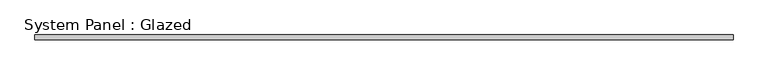
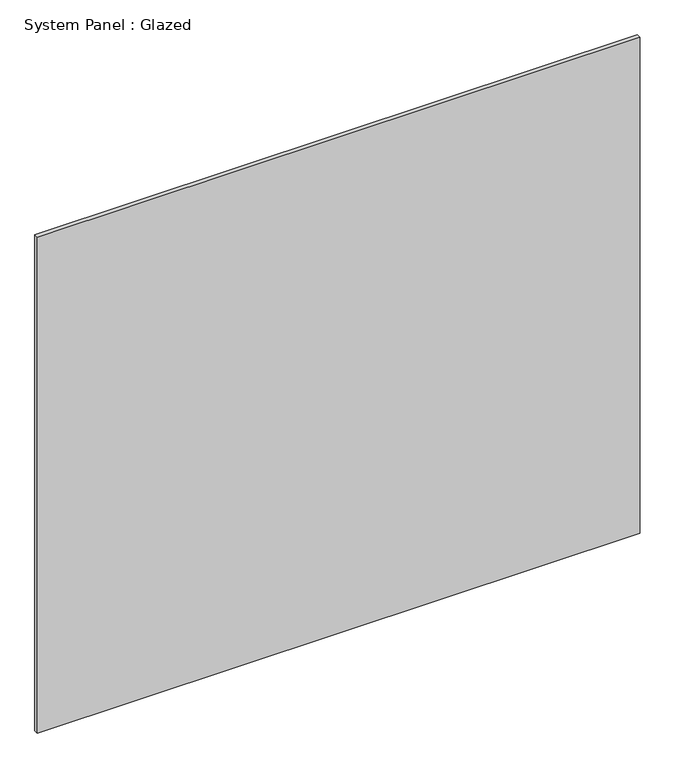
"""IFC4 building model written with IfcOpenShell, lengths in millimetres: plate geometry, System Panel : Glazed."""

from ifc_helpers import new_model, si_unit, origin, origin_with_axes, place, context, project, spatial, polyline, outline, extrude, source, transform, mapped, element, save


def system_panel_glazed_0ae67c42(model_context):
    return source(origin(), model_context, "Body", "SweptSolid", [
        extrude(outline(polyline([(1752.6, 19.05), (-1752.6, 19.05), (-1752.6, 44.45), (1752.6, 44.45), (1752.6, 19.05)])), origin_with_axes(), (0.0, 0.0, 1.0), 3048.0),
    ])


if __name__ == "__main__":
    model = new_model("IFC4")
    model_context = context("Model", 3, world=origin())
    ifc_project = project(units=[si_unit("LENGTHUNIT", "METRE", prefix="MILLI")], contexts=[model_context])
    site = spatial("IfcSite", under=ifc_project)
    building = spatial("IfcBuilding", under=site)
    placement = place(None, origin())
    system_panel_glazed_shape = system_panel_glazed_0ae67c42(model_context)
    element("IfcPlate", 1, ObjectType="System Panel : Glazed", at=placement, inside=building, context=model_context, shape_type="MappedRepresentation", body=[
        mapped(system_panel_glazed_shape, transform((0.0, 0.0, 0.0), x_axis=(1.0, 0.0, 0.0), y_axis=(0.0, 1.0, 0.0), z_axis=(0.0, 0.0, 1.0))),
    ])
    save(model, "model.ifc")

# Revit data of these elements
# Type "System Panel : Glazed"
#   Construction Type Id = "GSP4R"
#   Analytic Construction = "1/8 in Pilkington single glazing"
#   Visual Light Transmittance = 0.9
#   Solar Heat Gain Coefficient = 0.86
#   Heat Transfer Coefficient (U) = 1.18115 BTU/(h·ft²·°F)
#   Define Thermal Properties by = 1
# Element 1 (IfcPlate, "System Panel : Glazed")
#   Materials on its faces: "Glass"
# Materials
#   "Glass": class "Glass", colour RGB 0 128 192, transparency 0.75, Description = "Soda Lime Glass", Cost = 0
